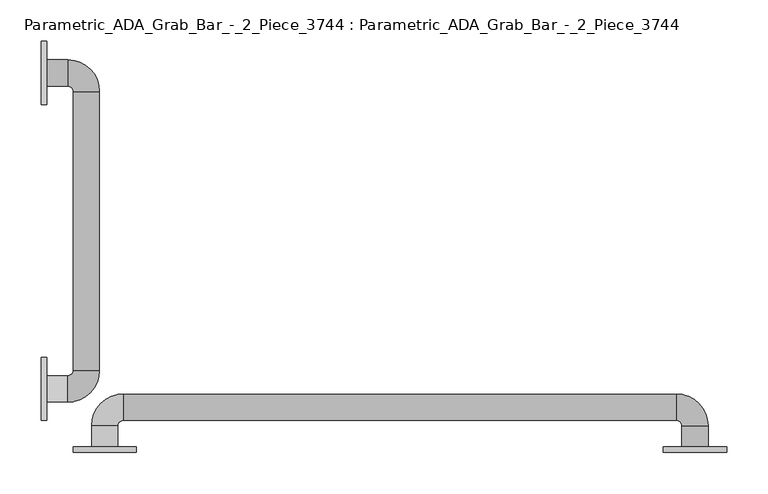
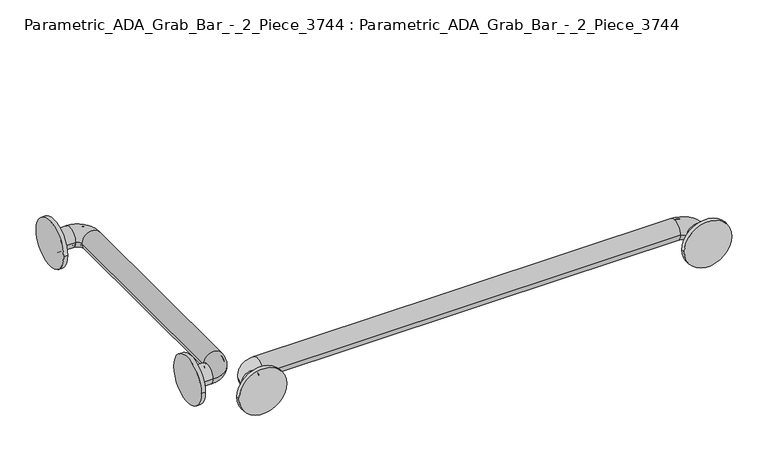
"""IFC4 building model written with IfcOpenShell, lengths in millimetres: proxy geometry, Parametric_ADA_Grab_Bar_-_2_Piece_3744 : Parametric_ADA_Grab_Bar_-_2_Piece_3744."""

import ifcopenshell
import ifcopenshell.guid

model = None  # the IFC model being written
_history = None  # IfcOwnerHistory: only IFC2X3 demands one
_inside = {}  # id of a spatial element -> (the spatial element, [elements in it])
_under = {}  # id of a project, library or spatial element -> (it, [spatial elements below it])
_declared = {}  # id of a project -> (the project, [libraries it declares])
_typed = {}  # id of a type object -> (the type object, [elements of that type])
_made_of = {}  # id of a material, layer set ... -> (it, [elements and type objects made of it])


def new_model(schema):
    """Start an empty IFC model of exactly this schema.

    Asked for "IFC4X3", IfcOpenShell would pick the latest addendum, in which some entities
    have other attributes; the version numbers below select the first issue.
    IFC2X3 requires an IfcOwnerHistory on every rooted entity: one is made here for all.
    """
    global model, _history
    if schema == "IFC4X3":
        model = ifcopenshell.file(schema_version=(4, 3, 0, 0))
    else:
        model = ifcopenshell.file(schema=schema)
    _inside.clear()
    _under.clear()
    _declared.clear()
    _typed.clear()
    _made_of.clear()
    _history = None
    if model.schema == "IFC2X3":
        org = make("IfcOrganization", Name="unknown")
        user = make(
            "IfcPersonAndOrganization",
            ThePerson=make("IfcPerson", FamilyName="unknown"),
            TheOrganization=org,
        )
        app = make(
            "IfcApplication",
            ApplicationDeveloper=org,
            Version="unknown",
            ApplicationFullName="unknown",
            ApplicationIdentifier="unknown",
        )
        _history = make(
            "IfcOwnerHistory",
            OwningUser=user,
            OwningApplication=app,
            ChangeAction="ADDED",
            CreationDate=0,
        )
    return model


def make(cls, **values):
    """One entity of the class cls with the attributes given. An attribute that is None is left unset."""
    return model.create_entity(
        cls, **{name: value for name, value in values.items() if value is not None}
    )


def rooted(cls, **values):
    """An entity with a GlobalId (a new one), such as an element, a storey or a relation."""
    return make(cls, GlobalId=ifcopenshell.guid.new(), OwnerHistory=_history, **values)


def si_unit(unit_type, name, prefix=None):
    """IfcSIUnit, for example si_unit("LENGTHUNIT", "METRE", prefix="MILLI")."""
    return make("IfcSIUnit", UnitType=unit_type, Prefix=prefix, Name=name)


def assignment(units):
    """IfcUnitAssignment: the units of a project."""
    return None if units is None else make("IfcUnitAssignment", Units=units)


def point(xyz):
    """IfcCartesianPoint."""
    return None if xyz is None else make("IfcCartesianPoint", Coordinates=xyz)


def direction(xyz):
    """IfcDirection."""
    return None if xyz is None else make("IfcDirection", DirectionRatios=xyz)


def frame(location, z_axis=None, x_axis=None):
    """IfcAxis2Placement3D, a coordinate frame: its origin and axes. An axis left out is left unset."""
    return make(
        "IfcAxis2Placement3D",
        Location=point(location),
        Axis=direction(z_axis),
        RefDirection=direction(x_axis),
    )


def frame_2d(location, x_axis=None):
    """IfcAxis2Placement2D, a coordinate frame in the plane: its origin and x axis."""
    return make(
        "IfcAxis2Placement2D", Location=point(location), RefDirection=direction(x_axis)
    )


def origin():
    """The frame at (0, 0, 0) with its axes left unset."""
    return frame((0.0, 0.0, 0.0))


def place(relative_to, where):
    """IfcLocalPlacement: puts the frame where relative to a parent placement (None: the world)."""
    return make(
        "IfcLocalPlacement", PlacementRelTo=relative_to, RelativePlacement=where
    )


def context(
    kind, dimensions, precision=None, world=None, true_north=None, identifier=None
):
    """IfcGeometricRepresentationContext, for example the 3D "Model" context."""
    return make(
        "IfcGeometricRepresentationContext",
        ContextIdentifier=identifier,
        ContextType=kind,
        CoordinateSpaceDimension=dimensions,
        Precision=precision,
        WorldCoordinateSystem=world,
        TrueNorth=true_north,
    )


def project(units=None, contexts=None):
    """IfcProject with its units and contexts."""
    return rooted(
        "IfcProject",
        Name="project",
        RepresentationContexts=contexts,
        UnitsInContext=assignment(units),
    )


def spatial(cls, under=None, at=None, **own):
    """A site, building, storey or space (cls), placed at a placement, below another one or the project."""
    s = rooted(cls, ObjectPlacement=at, **own)
    if under is not None:
        _under.setdefault(under.id(), (under, []))[1].append(s)
    return s


def polyline(points):
    """IfcPolyline through the points."""
    return make("IfcPolyline", Points=[point(p) for p in points])


def circle_curve(where, radius):
    """IfcCircle in the frame where."""
    return make("IfcCircle", Position=where, Radius=radius)


def ellipse_curve(where, semi_axis1, semi_axis2):
    """IfcEllipse in the frame where."""
    return make(
        "IfcEllipse", Position=where, SemiAxis1=semi_axis1, SemiAxis2=semi_axis2
    )


def trimmed(basis, trim1, trim2, sense, master):
    """IfcTrimmedCurve: the piece of a basis curve between two trims."""
    return make(
        "IfcTrimmedCurve",
        BasisCurve=basis,
        Trim1=trim1,
        Trim2=trim2,
        SenseAgreement=sense,
        MasterRepresentation=master,
    )


def segment(curve, same_sense, transition):
    """IfcCompositeCurveSegment."""
    return make(
        "IfcCompositeCurveSegment",
        Transition=transition,
        SameSense=same_sense,
        ParentCurve=curve,
    )


def composite_curve(segments, self_intersect=None):
    """IfcCompositeCurve: segments joined end to end."""
    return make("IfcCompositeCurve", Segments=segments, SelfIntersect=self_intersect)


def outline(outer, holes=None, kind="AREA"):
    """IfcArbitraryClosedProfileDef: a profile drawn as a closed curve; with holes, ...WithVoids."""
    if holes is None:
        return make("IfcArbitraryClosedProfileDef", ProfileType=kind, OuterCurve=outer)
    return make(
        "IfcArbitraryProfileDefWithVoids",
        ProfileType=kind,
        OuterCurve=outer,
        InnerCurves=holes,
    )


def extrude(swept, where, along, depth):
    """IfcExtrudedAreaSolid: the profile swept, set in the frame where, extruded along a direction by depth."""
    return make(
        "IfcExtrudedAreaSolid",
        SweptArea=swept,
        Position=where,
        ExtrudedDirection=direction(along),
        Depth=depth,
    )


def shape(context_of_items, identifier, shape_type, items):
    """IfcShapeRepresentation: the items that make up one representation, for example the "Body"."""
    return make(
        "IfcShapeRepresentation",
        ContextOfItems=context_of_items,
        RepresentationIdentifier=identifier,
        RepresentationType=shape_type,
        Items=items,
    )


def source(mapping_origin, context_of_items, identifier, shape_type, items):
    """IfcRepresentationMap: a shape defined once, which mapped items show again and again."""
    return make(
        "IfcRepresentationMap",
        MappingOrigin=mapping_origin,
        MappedRepresentation=shape(context_of_items, identifier, shape_type, items),
    )


def transform(
    local_origin,
    x_axis=None,
    y_axis=None,
    z_axis=None,
    scale=None,
    scale2=None,
    scale3=None,
    uniform=True,
):
    """IfcCartesianTransformationOperator3D, or its non-uniform kind. x_axis, y_axis, z_axis: its Axis1, 2, 3."""
    if uniform:
        return make(
            "IfcCartesianTransformationOperator3D",
            Axis1=direction(x_axis),
            Axis2=direction(y_axis),
            LocalOrigin=point(local_origin),
            Scale=scale,
            Axis3=direction(z_axis),
        )
    return make(
        "IfcCartesianTransformationOperator3DnonUniform",
        Axis1=direction(x_axis),
        Axis2=direction(y_axis),
        LocalOrigin=point(local_origin),
        Scale=scale,
        Axis3=direction(z_axis),
        Scale2=scale2,
        Scale3=scale3,
    )


def mapped(mapping_source, mapping_target):
    """IfcMappedItem: shows the shape of a source again, moved by a transform."""
    return make(
        "IfcMappedItem", MappingSource=mapping_source, MappingTarget=mapping_target
    )


def made_of(thing, what):
    """Note that an element or type object is made of a material, layer set ...; save() writes the relation."""
    if what is not None:
        _made_of.setdefault(what.id(), (what, []))[1].append(thing)
    return thing


def element(
    cls,
    number,
    at=None,
    inside=None,
    cuts=None,
    type_object=None,
    material=None,
    context=None,
    identifier="Body",
    shape_type=None,
    held_by="IfcProductDefinitionShape",
    body=None,
    shapes=None,
    **own,
):
    """One element of the class cls, such as IfcWall. Its Tag is "e" and its number.

    at: its placement. inside: the storey or other place that contains it. cuts: it is an
    opening in that element (IfcRelVoidsElement). A single representation is given by context,
    identifier, shape_type and body (its items); several are given by shapes. held_by: the class
    of the entity that holds the representations. save() writes the other relations.
    """
    e = rooted(cls, Tag="e%d" % number, ObjectPlacement=at, **own)
    if body is not None:
        shapes = [shape(context, identifier, shape_type, body)]
    if shapes is not None:
        e.Representation = make(held_by, Representations=shapes)
    if inside is not None:
        _inside.setdefault(inside.id(), (inside, []))[1].append(e)
    if cuts is not None:
        rooted(
            "IfcRelVoidsElement", RelatingBuildingElement=cuts, RelatedOpeningElement=e
        )
    if type_object is not None:
        _typed.setdefault(type_object.id(), (type_object, []))[1].append(e)
    return made_of(e, material)


def aggregate(whole, parts):
    """IfcRelAggregates: a whole, such as a stair, and the parts it consists of."""
    return rooted("IfcRelAggregates", RelatingObject=whole, RelatedObjects=parts)


def save(model, path):
    """Write the relations noted so far, then the file.

    IfcRelAggregates (storeys below a building ...), IfcRelContainedInSpatialStructure (elements
    in a storey), IfcRelDefinesByType, IfcRelAssociatesMaterial and IfcRelDeclares: one each for
    every whole, place, type object, material and project.
    """
    for whole, parts in _under.values():
        aggregate(whole, parts)
    for where, things in _inside.values():
        rooted(
            "IfcRelContainedInSpatialStructure",
            RelatedElements=things,
            RelatingStructure=where,
        )
    for kind, things in _typed.values():
        rooted("IfcRelDefinesByType", RelatedObjects=things, RelatingType=kind)
    for what, things in _made_of.values():
        rooted("IfcRelAssociatesMaterial", RelatedObjects=things, RelatingMaterial=what)
    for by, libraries in _declared.values():
        rooted("IfcRelDeclares", RelatingContext=by, RelatedDefinitions=libraries)
    model.write(path)


def plane_surface(at):
    """IfcPlane: the flat surface through the origin of the frame at, square to its z axis."""
    return make("IfcPlane", Position=at)


def cylinder_surface(at, radius):
    """IfcCylindricalSurface: all points at the distance radius from the z axis of the frame at."""
    return make("IfcCylindricalSurface", Position=at, Radius=radius)


def revolved_surface(curve, axis_point, axis_direction):
    """IfcSurfaceOfRevolution: the curve turned about the line through axis_point along axis_direction."""
    return make(
        "IfcSurfaceOfRevolution",
        SweptCurve=make("IfcArbitraryOpenProfileDef", ProfileType="CURVE", Curve=curve),
        AxisPosition=make("IfcAxis1Placement", Location=point(axis_point), Axis=direction(axis_direction)),
    )


def advanced_brep(points, edges, surfaces, faces):
    """IfcAdvancedBrep: a solid bounded by faces that lie on surfaces and meet in shared edges.

    An edge is (start, end): straight between two places in points (the first is 0);
    or (start, end, curve); or (start, end, curve, False) where it runs against its curve.
    A face is (place in surfaces, loops), or (place, loops, False) where it looks against
    its surface's normal. A loop lists edges by number (the first is 1), with a minus sign
    where the edge is run from its end to its start. The first loop is the outer one.
    """
    corners = [point(p) for p in points]
    vertices = [make("IfcVertexPoint", VertexGeometry=c) for c in corners]
    made = []
    for start, end, *more in edges:
        made.append(
            make(
                "IfcEdgeCurve",
                EdgeStart=vertices[start],
                EdgeEnd=vertices[end],
                EdgeGeometry=more[0] if more else make("IfcPolyline", Points=[corners[start], corners[end]]),
                SameSense=more[1] if len(more) > 1 else True,
            )
        )
    hull = []
    for where, loops, *sense in faces:
        bounds = []
        for j, loop in enumerate(loops):
            ring = [make("IfcOrientedEdge", EdgeElement=made[abs(k) - 1], Orientation=k > 0) for k in loop]
            bounds.append(
                make(
                    "IfcFaceOuterBound" if j == 0 else "IfcFaceBound",
                    Bound=make("IfcEdgeLoop", EdgeList=ring),
                    Orientation=True,
                )
            )
        hull.append(make("IfcAdvancedFace", Bounds=bounds, FaceSurface=surfaces[where], SameSense=sense[0] if sense else True))
    return make("IfcAdvancedBrep", Outer=make("IfcClosedShell", CfsFaces=hull))


def parametric_ada_grab_bar_2_piece_3744_parametric_ada_grab_bar_6f2753c4(model_context):
    return source(origin(), model_context, "Body", "SolidModel", [
        advanced_brep(
        [(6.35, 499.26875, 838.2), (6.35, 531.01875, 838.2), (6.35, 502.44375, 838.2), (6.35, 527.84375, 838.2), (31.75, 499.26875, 838.2), (31.75, 531.01875, 838.2), (31.75, 502.44375, 838.2), (31.75, 527.84375, 838.2), (69.85, 492.91875, 838.2), (38.1, 492.91875, 838.2), (66.675, 492.91875, 838.2), (41.275, 492.91875, 838.2), (38.1, 156.36875, 838.2), (69.85, 156.36875, 838.2), (41.275, 156.36875, 838.2), (66.675, 156.36875, 838.2), (31.75, 118.26875, 838.2), (31.75, 150.01875, 838.2), (31.75, 121.44375, 838.2), (31.75, 146.84375, 838.2), (6.35, 150.01875, 838.2), (6.35, 118.26875, 838.2), (6.35, 146.84375, 838.2), (6.35, 121.44375, 838.2)],
        [
            (0, 1, circle_curve(frame((6.35, 515.14375, 838.2), z_axis=(-1.0, 0.0, 0.0), x_axis=(0.0, 1.0, 0.0)), 15.875)),
            (1, 0, circle_curve(frame((6.35, 515.14375, 838.2), z_axis=(-1.0, 0.0, 0.0), x_axis=(0.0, 1.0, 0.0)), 15.875)),
            (2, 3, circle_curve(frame((6.35, 515.14375, 838.2), z_axis=(1.0, 0.0, 0.0), x_axis=(0.0, 1.0, 0.0)), 12.7)),
            (3, 2, circle_curve(frame((6.35, 515.14375, 838.2), z_axis=(1.0, 0.0, 0.0), x_axis=(0.0, 1.0, 0.0)), 12.7)),
            (0, 4),
            (4, 5, circle_curve(frame((31.75, 515.14375, 838.2), z_axis=(-1.0, 0.0, 0.0), x_axis=(0.0, 1.0, 0.0)), 15.875)),
            (5, 1),
            (5, 4, circle_curve(frame((31.75, 515.14375, 838.2), z_axis=(-1.0, 0.0, 0.0), x_axis=(0.0, 1.0, 0.0)), 15.875)),
            (2, 6),
            (6, 7, circle_curve(frame((31.75, 515.14375, 838.2), z_axis=(1.0, 0.0, 0.0), x_axis=(0.0, 1.0, 0.0)), 12.7)),
            (7, 3),
            (7, 6, circle_curve(frame((31.75, 515.14375, 838.2), z_axis=(1.0, 0.0, 0.0), x_axis=(0.0, 1.0, 0.0)), 12.7)),
            (8, 5, circle_curve(frame((31.75, 492.91875, 838.2), z_axis=(0.0, 0.0, 1.0), x_axis=(0.0, 1.0, 0.0)), 38.1)),
            (4, 9, circle_curve(frame((31.75, 492.91875, 838.2), z_axis=(0.0, 0.0, -1.0), x_axis=(0.0, 1.0, 0.0)), 6.35)),
            (9, 8, circle_curve(frame((53.975, 492.91875, 838.2), z_axis=(0.0, 1.0, 0.0), x_axis=(1.0, 0.0, 0.0)), 15.875)),
            (8, 9, circle_curve(frame((53.975, 492.91875, 838.2), z_axis=(0.0, 1.0, 0.0), x_axis=(1.0, 0.0, 0.0)), 15.875)),
            (10, 7, circle_curve(frame((31.75, 492.91875, 838.2), z_axis=(0.0, 0.0, 1.0), x_axis=(0.0, 1.0, 0.0)), 34.925)),
            (6, 11, circle_curve(frame((31.75, 492.91875, 838.2), z_axis=(0.0, 0.0, -1.0), x_axis=(0.0, 1.0, 0.0)), 9.525)),
            (11, 10, circle_curve(frame((53.975, 492.91875, 838.2), z_axis=(0.0, -1.0, 0.0), x_axis=(1.0, 0.0, 0.0)), 12.7)),
            (10, 11, circle_curve(frame((53.975, 492.91875, 838.2), z_axis=(0.0, -1.0, 0.0), x_axis=(1.0, 0.0, 0.0)), 12.7)),
            (9, 12),
            (12, 13, circle_curve(frame((53.975, 156.36875, 838.2), z_axis=(0.0, 1.0, 0.0), x_axis=(1.0, 0.0, 0.0)), 15.875)),
            (13, 8),
            (13, 12, circle_curve(frame((53.975, 156.36875, 838.2), z_axis=(0.0, 1.0, 0.0), x_axis=(1.0, 0.0, 0.0)), 15.875)),
            (11, 14),
            (14, 15, circle_curve(frame((53.975, 156.36875, 838.2), z_axis=(0.0, -1.0, 0.0), x_axis=(1.0, 0.0, 0.0)), 12.7)),
            (15, 10),
            (15, 14, circle_curve(frame((53.975, 156.36875, 838.2), z_axis=(0.0, -1.0, 0.0), x_axis=(1.0, 0.0, 0.0)), 12.7)),
            (16, 13, circle_curve(frame((31.75, 156.36875, 838.2), z_axis=(0.0, 0.0, 1.0), x_axis=(1.0, 0.0, 0.0)), 38.1)),
            (12, 17, circle_curve(frame((31.75, 156.36875, 838.2), z_axis=(0.0, 0.0, -1.0), x_axis=(1.0, 0.0, 0.0)), 6.35)),
            (17, 16, circle_curve(frame((31.75, 134.14375, 838.2), z_axis=(1.0, -1.0754999491619899e-12, 0.0), x_axis=(-1.0754999491619899e-12, -1.0, 0.0)), 15.875)),
            (16, 17, circle_curve(frame((31.75, 134.14375, 838.2), z_axis=(1.0, 0.0, 0.0), x_axis=(0.0, -1.0, 0.0)), 15.875)),
            (18, 15, circle_curve(frame((31.75, 156.36875, 838.2), z_axis=(0.0, 0.0, 1.0), x_axis=(1.0, 0.0, 0.0)), 34.925)),
            (14, 19, circle_curve(frame((31.75, 156.36875, 838.2), z_axis=(0.0, 0.0, -1.0), x_axis=(1.0, 0.0, 0.0)), 9.525)),
            (19, 18, circle_curve(frame((31.75, 134.14375, 838.2), z_axis=(-1.0, 0.0, 0.0), x_axis=(0.0, -1.0, 0.0)), 12.7)),
            (18, 19, circle_curve(frame((31.75, 134.14375, 838.2), z_axis=(-1.0, 0.0, 0.0), x_axis=(0.0, -1.0, 0.0)), 12.7)),
            (20, 21, circle_curve(frame((6.35, 134.14375, 838.2), z_axis=(-1.0, 0.0, 0.0), x_axis=(0.0, -1.0, 0.0)), 15.875)),
            (21, 20, circle_curve(frame((6.35, 134.14375, 838.2), z_axis=(-1.0, 0.0, 0.0), x_axis=(0.0, -1.0, 0.0)), 15.875)),
            (22, 23, circle_curve(frame((6.35, 134.14375, 838.2), z_axis=(1.0, 0.0, 0.0), x_axis=(0.0, -1.0, 0.0)), 12.7)),
            (23, 22, circle_curve(frame((6.35, 134.14375, 838.2), z_axis=(1.0, 0.0, 0.0), x_axis=(0.0, -1.0, 0.0)), 12.7)),
            (17, 20),
            (21, 16),
            (19, 22),
            (23, 18),
        ],
        [
            plane_surface(frame((6.35, 515.14375, 838.2), z_axis=(-1.0, 0.0, 0.0), x_axis=(0.0, 0.0, 1.0))),
            cylinder_surface(frame((6.35, 515.14375, 838.2), z_axis=(-1.0, 0.0, 0.0), x_axis=(0.0, 1.0, 0.0)), 15.875),
            revolved_surface(polyline([(31.75, 527.84375, 838.2), (6.35, 527.84375, 838.2)]), (6.35, 515.14375, 838.2), (1.0, 0.0, 0.0)),
            revolved_surface(trimmed(ellipse_curve(frame((31.75, 515.14375, 838.2), z_axis=(-1.0, 0.0, 0.0), x_axis=(0.0, 1.0, 0.0)), 15.875, 15.875), [point((31.75, 499.26875, 838.2))], [point((31.75, 531.01875, 838.2))], True, "CARTESIAN"), (31.75, 492.91875, 838.2), (0.0, 0.0, -1.0)),
            revolved_surface(trimmed(ellipse_curve(frame((31.75, 515.14375, 838.2), z_axis=(-1.0, 0.0, 0.0), x_axis=(0.0, 1.0, 0.0)), 15.875, 15.875), [point((31.75, 531.01875, 838.2))], [point((31.75, 499.26875, 838.2))], True, "CARTESIAN"), (31.75, 492.91875, 838.2), (0.0, 0.0, -1.0)),
            revolved_surface(trimmed(ellipse_curve(frame((31.75, 515.14375, 838.2), z_axis=(1.0, 0.0, 0.0), x_axis=(0.0, 1.0, 0.0)), 12.7, 12.7), [point((31.75, 502.44375, 838.2))], [point((31.75, 527.84375, 838.2))], True, "CARTESIAN"), (31.75, 492.91875, 838.2), (0.0, 0.0, -1.0)),
            revolved_surface(trimmed(ellipse_curve(frame((31.75, 515.14375, 838.2), z_axis=(1.0, 0.0, 0.0), x_axis=(0.0, 1.0, 0.0)), 12.7, 12.7), [point((31.75, 527.84375, 838.2))], [point((31.75, 502.44375, 838.2))], True, "CARTESIAN"), (31.75, 492.91875, 838.2), (0.0, 0.0, -1.0)),
            cylinder_surface(frame((53.975, 492.91875, 838.2), z_axis=(0.0, 1.0, 0.0), x_axis=(1.0, 0.0, 0.0)), 15.875),
            revolved_surface(polyline([(66.675, 156.36875000000003, 838.2), (66.675, 492.91875, 838.2)]), (53.975, 492.91875, 838.2), (0.0, -1.0, 0.0)),
            revolved_surface(trimmed(ellipse_curve(frame((53.975, 156.36875, 838.2), z_axis=(0.0, 1.0, 0.0), x_axis=(1.0, 0.0, 0.0)), 15.875, 15.875), [point((38.1, 156.36875, 838.2))], [point((69.85, 156.36875, 838.2))], True, "CARTESIAN"), (31.75, 156.36875, 838.2), (0.0, 0.0, -1.0)),
            revolved_surface(trimmed(ellipse_curve(frame((53.975, 156.36875, 838.2), z_axis=(0.0, 1.0, 0.0), x_axis=(1.0, 0.0, 0.0)), 15.875, 15.875), [point((69.85, 156.36875, 838.2))], [point((38.1, 156.36875, 838.2))], True, "CARTESIAN"), (31.75, 156.36875, 838.2), (0.0, 0.0, -1.0)),
            revolved_surface(trimmed(ellipse_curve(frame((53.975, 156.36875, 838.2), z_axis=(0.0, -1.0, 0.0), x_axis=(1.0, 0.0, 0.0)), 12.7, 12.7), [point((41.275, 156.36875, 838.2))], [point((66.675, 156.36875, 838.2))], True, "CARTESIAN"), (31.75, 156.36875, 838.2), (0.0, 0.0, -1.0)),
            revolved_surface(trimmed(ellipse_curve(frame((53.975, 156.36875, 838.2), z_axis=(0.0, -1.0, 0.0), x_axis=(1.0, 0.0, 0.0)), 12.7, 12.7), [point((66.675, 156.36875, 838.2))], [point((41.275, 156.36875, 838.2))], True, "CARTESIAN"), (31.75, 156.36875, 838.2), (0.0, 0.0, -1.0)),
            plane_surface(frame((6.35, 134.14375, 838.2), z_axis=(-1.0, 0.0, 0.0), x_axis=(0.0, 0.0, 1.0))),
            cylinder_surface(frame((31.75, 134.14375, 838.2), z_axis=(1.0, 0.0, 0.0), x_axis=(0.0, -1.0, 0.0)), 15.875),
            revolved_surface(polyline([(6.350000000000001, 121.44375000000001, 838.2), (31.75, 121.44375000000001, 838.2)]), (31.75, 134.14375, 838.2), (-1.0, 0.0, 0.0)),
        ],
        [
            (0, [[1, 2], [3, 4]]),
            (1, [[-1, 5, 6, 7]]),
            (1, [[-2, -7, 8, -5]]),
            (2, [[-3, 9, 10, 11]]),
            (2, [[-4, -11, 12, -9]]),
            (3, [[13, -6, 14, 15]]),
            (4, [[-14, -8, -13, 16]]),
            (5, [[17, -10, 18, 19]]),
            (6, [[-18, -12, -17, 20]]),
            (7, [[-15, 21, 22, 23]]),
            (7, [[-16, -23, 24, -21]]),
            (8, [[-19, 25, 26, 27]]),
            (8, [[-20, -27, 28, -25]]),
            (9, [[29, -22, 30, 31]]),
            (10, [[-30, -24, -29, 32]]),
            (11, [[33, -26, 34, 35]]),
            (12, [[-34, -28, -33, 36]]),
            (13, [[37, 38], [39, 40]]),
            (14, [[-31, 41, -38, 42]]),
            (14, [[-32, -42, -37, -41]]),
            (15, [[-35, 43, -40, 44]]),
            (15, [[-36, -44, -39, -43]]),
        ],
    ),
        advanced_brep(
        [(92.075, 64.29375, 838.2), (60.325, 64.29375, 838.2), (88.9, 64.29375, 838.2), (63.5, 64.29375, 838.2), (92.075, 89.69375, 838.2), (60.325, 89.69375, 838.2), (88.9, 89.69375, 838.2), (63.5, 89.69375, 838.2), (98.425, 127.79375, 838.2), (98.425, 96.04375, 838.2), (98.425, 124.61875, 838.2), (98.425, 99.21875, 838.2), (765.175, 96.04375, 838.2), (765.175, 127.79375, 838.2), (765.175, 99.21875, 838.2), (765.175, 124.61875, 838.2), (803.275, 89.69375, 838.2), (771.525, 89.69375, 838.2), (800.1, 89.69375, 838.2), (774.7, 89.69375, 838.2), (771.525, 64.29375, 838.2), (803.275, 64.29375, 838.2), (774.7, 64.29375, 838.2), (800.1, 64.29375, 838.2)],
        [
            (0, 1, circle_curve(frame((76.2, 64.29375, 838.2), z_axis=(0.0, -1.0, 0.0), x_axis=(-1.0, 0.0, 0.0)), 15.875)),
            (1, 0, circle_curve(frame((76.2, 64.29375, 838.2), z_axis=(0.0, -1.0, 0.0), x_axis=(-1.0, 0.0, 0.0)), 15.875)),
            (2, 3, circle_curve(frame((76.2, 64.29375, 838.2), z_axis=(0.0, 1.0, 0.0), x_axis=(-1.0, 0.0, 0.0)), 12.7)),
            (3, 2, circle_curve(frame((76.2, 64.29375, 838.2), z_axis=(0.0, 1.0, 0.0), x_axis=(-1.0, 0.0, 0.0)), 12.7)),
            (0, 4),
            (4, 5, circle_curve(frame((76.2, 89.69375, 838.2), z_axis=(0.0, -1.0, 0.0), x_axis=(-1.0, 0.0, 0.0)), 15.875)),
            (5, 1),
            (5, 4, circle_curve(frame((76.2, 89.69375, 838.2), z_axis=(0.0, -1.0, 0.0), x_axis=(-1.0, 0.0, 0.0)), 15.875)),
            (2, 6),
            (6, 7, circle_curve(frame((76.2, 89.69375, 838.2), z_axis=(0.0, 1.0, 0.0), x_axis=(-1.0, 0.0, 0.0)), 12.7)),
            (7, 3),
            (7, 6, circle_curve(frame((76.2, 89.69375, 838.2), z_axis=(0.0, 1.0, 0.0), x_axis=(-1.0, 0.0, 0.0)), 12.7)),
            (8, 5, circle_curve(frame((98.425, 89.69375, 838.2), z_axis=(0.0, 0.0, 1.0), x_axis=(-1.0, 0.0, 0.0)), 38.1)),
            (4, 9, circle_curve(frame((98.425, 89.69375, 838.2), z_axis=(0.0, 0.0, -1.0), x_axis=(-1.0, 0.0, 0.0)), 6.35)),
            (9, 8, circle_curve(frame((98.425, 111.91875, 838.2), z_axis=(-1.0, 0.0, 0.0), x_axis=(0.0, 1.0, 0.0)), 15.875)),
            (8, 9, circle_curve(frame((98.425, 111.91875, 838.2), z_axis=(-1.0, 0.0, 0.0), x_axis=(0.0, 1.0, 0.0)), 15.875)),
            (10, 7, circle_curve(frame((98.425, 89.69375, 838.2), z_axis=(0.0, 0.0, 1.0), x_axis=(-1.0, 0.0, 0.0)), 34.925)),
            (6, 11, circle_curve(frame((98.425, 89.69375, 838.2), z_axis=(0.0, 0.0, -1.0), x_axis=(-1.0, 0.0, 0.0)), 9.525)),
            (11, 10, circle_curve(frame((98.425, 111.91875, 838.2), z_axis=(1.0, 0.0, 0.0), x_axis=(0.0, 1.0, 0.0)), 12.7)),
            (10, 11, circle_curve(frame((98.425, 111.91875, 838.2), z_axis=(1.0, 0.0, 0.0), x_axis=(0.0, 1.0, 0.0)), 12.7)),
            (9, 12),
            (12, 13, circle_curve(frame((765.175, 111.91875, 838.2), z_axis=(-1.0, 0.0, 0.0), x_axis=(0.0, 1.0, 0.0)), 15.875)),
            (13, 8),
            (13, 12, circle_curve(frame((765.175, 111.91875, 838.2), z_axis=(-1.0, 0.0, 0.0), x_axis=(0.0, 1.0, 0.0)), 15.875)),
            (11, 14),
            (14, 15, circle_curve(frame((765.175, 111.91875, 838.2), z_axis=(1.0, 0.0, 0.0), x_axis=(0.0, 1.0, 0.0)), 12.7)),
            (15, 10),
            (15, 14, circle_curve(frame((765.175, 111.91875, 838.2), z_axis=(1.0, 0.0, 0.0), x_axis=(0.0, 1.0, 0.0)), 12.7)),
            (16, 13, circle_curve(frame((765.175, 89.69375, 838.2), z_axis=(0.0, 0.0, 1.0), x_axis=(0.0, 1.0, 0.0)), 38.1)),
            (12, 17, circle_curve(frame((765.175, 89.69375, 838.2), z_axis=(0.0, 0.0, -1.0), x_axis=(0.0, 1.0, 0.0)), 6.35)),
            (17, 16, circle_curve(frame((787.4, 89.69375, 838.2), z_axis=(1.0770542613964651e-12, 1.0, 0.0), x_axis=(1.0, -1.0770542613964651e-12, 0.0)), 15.875)),
            (16, 17, circle_curve(frame((787.4, 89.69375, 838.2), z_axis=(0.0, 1.0, 0.0), x_axis=(1.0, 0.0, 0.0)), 15.875)),
            (18, 15, circle_curve(frame((765.175, 89.69375, 838.2), z_axis=(0.0, 0.0, 1.0), x_axis=(0.0, 1.0, 0.0)), 34.925)),
            (14, 19, circle_curve(frame((765.175, 89.69375, 838.2), z_axis=(0.0, 0.0, -1.0), x_axis=(0.0, 1.0, 0.0)), 9.525)),
            (19, 18, circle_curve(frame((787.4, 89.69375, 838.2), z_axis=(0.0, -1.0, 0.0), x_axis=(1.0, 0.0, 0.0)), 12.7)),
            (18, 19, circle_curve(frame((787.4, 89.69375, 838.2), z_axis=(0.0, -1.0, 0.0), x_axis=(1.0, 0.0, 0.0)), 12.7)),
            (20, 21, circle_curve(frame((787.4, 64.29375, 838.2), z_axis=(0.0, -1.0, 0.0), x_axis=(1.0, 0.0, 0.0)), 15.875)),
            (21, 20, circle_curve(frame((787.4, 64.29375, 838.2), z_axis=(0.0, -1.0, 0.0), x_axis=(1.0, 0.0, 0.0)), 15.875)),
            (22, 23, circle_curve(frame((787.4, 64.29375, 838.2), z_axis=(0.0, 1.0, 0.0), x_axis=(1.0, 0.0, 0.0)), 12.7)),
            (23, 22, circle_curve(frame((787.4, 64.29375, 838.2), z_axis=(0.0, 1.0, 0.0), x_axis=(1.0, 0.0, 0.0)), 12.7)),
            (17, 20),
            (21, 16),
            (19, 22),
            (23, 18),
        ],
        [
            plane_surface(frame((76.2, 64.29375, 838.2), z_axis=(0.0, -1.0, 0.0), x_axis=(0.0, 0.0, 1.0))),
            cylinder_surface(frame((76.2, 64.29375, 838.2), z_axis=(0.0, -1.0, 0.0), x_axis=(-1.0, 0.0, 0.0)), 15.875),
            revolved_surface(polyline([(63.5, 89.69375, 838.2), (63.5, 64.29375, 838.2)]), (76.2, 64.29375, 838.2), (0.0, 1.0, 0.0)),
            revolved_surface(trimmed(ellipse_curve(frame((76.2, 89.69375, 838.2), z_axis=(0.0, -1.0, 0.0), x_axis=(-1.0, 0.0, 0.0)), 15.875, 15.875), [point((92.075, 89.69375, 838.2))], [point((60.325, 89.69375, 838.2))], True, "CARTESIAN"), (98.425, 89.69375, 838.2), (0.0, 0.0, -1.0)),
            revolved_surface(trimmed(ellipse_curve(frame((76.2, 89.69375, 838.2), z_axis=(0.0, -1.0, 0.0), x_axis=(-1.0, 0.0, 0.0)), 15.875, 15.875), [point((60.325, 89.69375, 838.2))], [point((92.075, 89.69375, 838.2))], True, "CARTESIAN"), (98.425, 89.69375, 838.2), (0.0, 0.0, -1.0)),
            revolved_surface(trimmed(ellipse_curve(frame((76.2, 89.69375, 838.2), z_axis=(0.0, 1.0, 0.0), x_axis=(-1.0, 0.0, 0.0)), 12.7, 12.7), [point((88.9, 89.69375, 838.2))], [point((63.5, 89.69375, 838.2))], True, "CARTESIAN"), (98.425, 89.69375, 838.2), (0.0, 0.0, -1.0)),
            revolved_surface(trimmed(ellipse_curve(frame((76.2, 89.69375, 838.2), z_axis=(0.0, 1.0, 0.0), x_axis=(-1.0, 0.0, 0.0)), 12.7, 12.7), [point((63.5, 89.69375, 838.2))], [point((88.9, 89.69375, 838.2))], True, "CARTESIAN"), (98.425, 89.69375, 838.2), (0.0, 0.0, -1.0)),
            cylinder_surface(frame((98.425, 111.91875, 838.2), z_axis=(-1.0, 0.0, 0.0), x_axis=(0.0, 1.0, 0.0)), 15.875),
            revolved_surface(polyline([(765.175, 124.61875, 838.2), (98.425, 124.61875, 838.2)]), (98.425, 111.91875, 838.2), (1.0, 0.0, 0.0)),
            revolved_surface(trimmed(ellipse_curve(frame((765.175, 111.91875, 838.2), z_axis=(-1.0, 0.0, 0.0), x_axis=(0.0, 1.0, 0.0)), 15.875, 15.875), [point((765.175, 96.04375, 838.2))], [point((765.175, 127.79375, 838.2))], True, "CARTESIAN"), (765.175, 89.69375, 838.2), (0.0, 0.0, -1.0)),
            revolved_surface(trimmed(ellipse_curve(frame((765.175, 111.91875, 838.2), z_axis=(-1.0, 0.0, 0.0), x_axis=(0.0, 1.0, 0.0)), 15.875, 15.875), [point((765.175, 127.79375, 838.2))], [point((765.175, 96.04375, 838.2))], True, "CARTESIAN"), (765.175, 89.69375, 838.2), (0.0, 0.0, -1.0)),
            revolved_surface(trimmed(ellipse_curve(frame((765.175, 111.91875, 838.2), z_axis=(1.0, 0.0, 0.0), x_axis=(0.0, 1.0, 0.0)), 12.7, 12.7), [point((765.175, 99.21875, 838.2))], [point((765.175, 124.61875, 838.2))], True, "CARTESIAN"), (765.175, 89.69375, 838.2), (0.0, 0.0, -1.0)),
            revolved_surface(trimmed(ellipse_curve(frame((765.175, 111.91875, 838.2), z_axis=(1.0, 0.0, 0.0), x_axis=(0.0, 1.0, 0.0)), 12.7, 12.7), [point((765.175, 124.61875, 838.2))], [point((765.175, 99.21875, 838.2))], True, "CARTESIAN"), (765.175, 89.69375, 838.2), (0.0, 0.0, -1.0)),
            plane_surface(frame((787.4, 64.29375, 838.2), z_axis=(0.0, -1.0, 0.0), x_axis=(0.0, 0.0, 1.0))),
            cylinder_surface(frame((787.4, 89.69375, 838.2), z_axis=(0.0, 1.0, 0.0), x_axis=(1.0, 0.0, 0.0)), 15.875),
            revolved_surface(polyline([(800.1, 64.29375, 838.2), (800.1, 89.69375, 838.2)]), (787.4, 89.69375, 838.2), (0.0, -1.0, 0.0)),
        ],
        [
            (0, [[1, 2], [3, 4]]),
            (1, [[-1, 5, 6, 7]]),
            (1, [[-2, -7, 8, -5]]),
            (2, [[-3, 9, 10, 11]]),
            (2, [[-4, -11, 12, -9]]),
            (3, [[13, -6, 14, 15]]),
            (4, [[-14, -8, -13, 16]]),
            (5, [[17, -10, 18, 19]]),
            (6, [[-18, -12, -17, 20]]),
            (7, [[-15, 21, 22, 23]]),
            (7, [[-16, -23, 24, -21]]),
            (8, [[-19, 25, 26, 27]]),
            (8, [[-20, -27, 28, -25]]),
            (9, [[29, -22, 30, 31]]),
            (10, [[-30, -24, -29, 32]]),
            (11, [[33, -26, 34, 35]]),
            (12, [[-34, -28, -33, 36]]),
            (13, [[37, 38], [39, 40]]),
            (14, [[-31, 41, -38, 42]]),
            (14, [[-32, -42, -37, -41]]),
            (15, [[-35, 43, -40, 44]]),
            (15, [[-36, -44, -39, -43]]),
        ],
    ),
        extrude(outline(composite_curve([segment(trimmed(circle_curve(frame_2d((134.14375, 838.2)), 38.1), [point((96.04375, 838.2))], [point((172.24375, 838.2))], False, "CARTESIAN"), True, "CONTINUOUS"), segment(trimmed(circle_curve(frame_2d((134.14375, 838.2)), 38.1), [point((172.24375, 838.2))], [point((96.04375, 838.2))], False, "CARTESIAN"), True, "CONTINUOUS")], self_intersect=False)), frame((0.0, 0.0, 0.0), z_axis=(1.0, 0.0, 0.0), x_axis=(0.0, 1.0, 0.0)), (0.0, 0.0, 1.0), 6.35),
        extrude(outline(composite_curve([segment(trimmed(circle_curve(frame_2d((515.14375, 838.2)), 38.1), [point((477.04375, 838.2))], [point((553.24375, 838.2))], False, "CARTESIAN"), True, "CONTINUOUS"), segment(trimmed(circle_curve(frame_2d((515.14375, 838.2)), 38.1), [point((553.24375, 838.2))], [point((477.04375, 838.2))], False, "CARTESIAN"), True, "CONTINUOUS")], self_intersect=False)), frame((0.0, 0.0, 0.0), z_axis=(1.0, 0.0, 0.0), x_axis=(0.0, 1.0, 0.0)), (0.0, 0.0, 1.0), 6.35),
        extrude(outline(composite_curve([segment(trimmed(circle_curve(frame_2d((838.2, 787.4)), 38.1), [point((838.2, 749.3))], [point((838.2, 825.5))], False, "CARTESIAN"), True, "CONTINUOUS"), segment(trimmed(circle_curve(frame_2d((838.2, 787.4)), 38.1), [point((838.2, 825.5))], [point((838.2, 749.3))], False, "CARTESIAN"), True, "CONTINUOUS")], self_intersect=False)), frame((0.0, 57.94375, 0.0), z_axis=(0.0, 1.0, 0.0), x_axis=(0.0, 0.0, 1.0)), (0.0, 0.0, 1.0), 6.35),
        extrude(outline(composite_curve([segment(trimmed(circle_curve(frame_2d((838.2, 76.2)), 38.1), [point((838.2, 38.1))], [point((838.2, 114.3))], False, "CARTESIAN"), True, "CONTINUOUS"), segment(trimmed(circle_curve(frame_2d((838.2, 76.2)), 38.1), [point((838.2, 114.3))], [point((838.2, 38.1))], False, "CARTESIAN"), True, "CONTINUOUS")], self_intersect=False)), frame((0.0, 57.94375, 0.0), z_axis=(0.0, 1.0, 0.0), x_axis=(0.0, 0.0, 1.0)), (0.0, 0.0, 1.0), 6.35),
    ])


if __name__ == "__main__":
    model = new_model("IFC4")
    model_context = context("Model", 3, world=origin())
    ifc_project = project(units=[si_unit("LENGTHUNIT", "METRE", prefix="MILLI")], contexts=[model_context])
    site = spatial("IfcSite", under=ifc_project)
    building = spatial("IfcBuilding", under=site)
    placement = place(None, origin())
    parametric_ada_grab_bar_2_piece_3744_parametric_ada_grab_bar_shape = parametric_ada_grab_bar_2_piece_3744_parametric_ada_grab_bar_6f2753c4(model_context)
    element("IfcBuildingElementProxy", 1, Name="Parametric_ADA_Grab_Bar_-_2_Piece_3744 : Parametric_ADA_Grab_Bar_-_2_Piece_3744", ObjectType="Parametric_ADA_Grab_Bar_-_2_Piece_3744 : Parametric_ADA_Grab_Bar_-_2_Piece_3744", at=placement, inside=building, context=model_context, shape_type="MappedRepresentation", body=[
        mapped(parametric_ada_grab_bar_2_piece_3744_parametric_ada_grab_bar_shape, transform((0.0, 0.0, 0.0), x_axis=(1.0, 0.0, 0.0), y_axis=(0.0, 1.0, 0.0), z_axis=(0.0, 0.0, 1.0))),
    ])
    save(model, "model.ifc")

# Revit data of these elements
# Type "Parametric_ADA_Grab_Bar_-_2_Piece_3744 : Parametric_ADA_Grab_Bar_-_2_Piece_3744"
#   Keynote = "M10281313.01"
#   Grab bar length (42" min) = 1' - 3"
#   Grab bar height = 2' - 9"
#   Grab bar Length (36" min) = 2' - 4"
#   Face of Wall to Grab bar (6" max) = 0' - 3"
#   Face of Wall to Grab bar (12" max) = 0' - 3"
# Element 1 (IfcBuildingElementProxy, "Parametric_ADA_Grab_Bar_-_2_Piece_3744 : Parametric_ADA_Grab_Bar_-_2_Piece_3744")
#   Materials on its faces: "Stainless Steel"
# Materials
#   "Stainless Steel": class "Metal", colour RGB 0 0 0, transparency 0, Description = "Stainless Steel 18/8", Cost = 0
